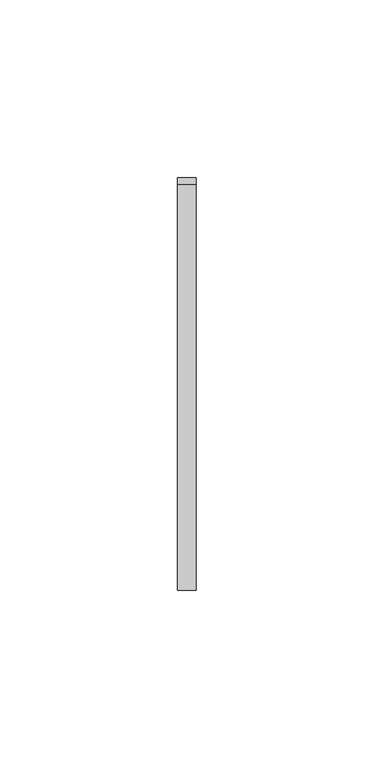
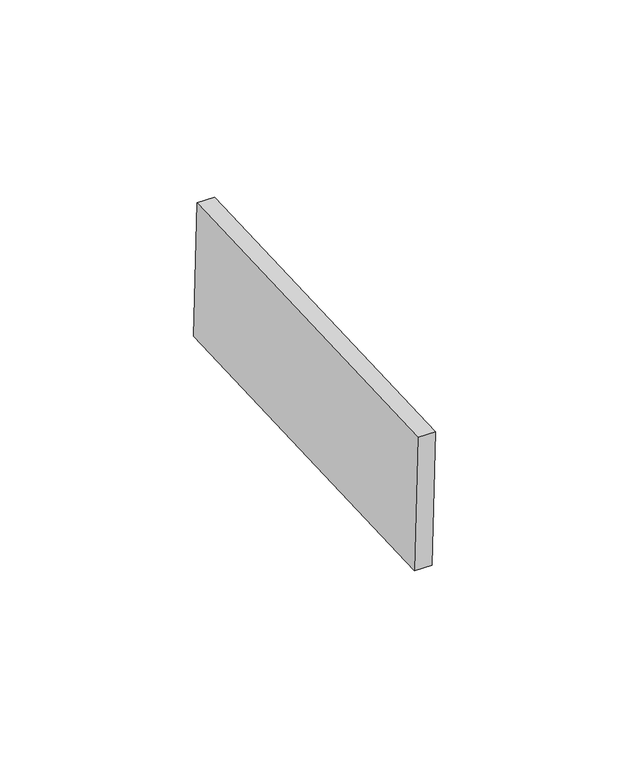
"""IFC4 building model written with IfcOpenShell, lengths in millimetres: proxy geometry, Inner panel:Inner panel:1:Inner panel:1 : Inner panel:Inner panel:300324:2:Inner panel:1:Inner panel:1 : Inner panel:Inner panel:300324:2 : Inner panel:Inner panel:1:Inner panel:1 : Inner panel:Inner panel:300324:300043:65 : Inner panel:Inner panel:1:Inner panel:1 : Inner panel:Inner panel:300324:2:Inner panel:1:Inner panel:1 : Inner panel:Inner panel:300324:2 : Inner panel:Inner panel:1:Inner panel:1 : Inner panel:Inner panel:300324:300043:308120."""

from ifc_helpers import new_model, si_unit, frame, origin, place, context, project, spatial, polyline, outline, extrude, source, transform, mapped, element, save


def generic_models_1821906e(model_context):
    return source(origin(), model_context, "Body", "SweptSolid", [
        extrude(outline(polyline([(0.0, -114.2999999), (0.0, 0.0), (5.2138089, 0.0), (5.2138089, -114.2999999), (0.0, -114.2999999)])), frame((593530.195117, -569718.1460118, 8742.3617848), z_axis=(0.0, -0.04163054471215927, 0.9991330730923529), x_axis=(-1.0, 0.0, 0.0)), (0.0, 0.0, 1.0), 43.2233908),
    ])


if __name__ == "__main__":
    model = new_model("IFC4")
    model_context = context("Model", 3, world=origin())
    ifc_project = project(units=[si_unit("LENGTHUNIT", "METRE", prefix="MILLI")], contexts=[model_context])
    site = spatial("IfcSite", under=ifc_project)
    building = spatial("IfcBuilding", under=site)
    placement = place(None, origin())
    generic_models_shape = generic_models_1821906e(model_context)
    element("IfcBuildingElementProxy", 1, Name="Inner panel:Inner panel:1:Inner panel:1 : Inner panel:Inner panel:300324:2:Inner panel:1:Inner panel:1 : Inner panel:Inner panel:300324:2 : Inner panel:Inner panel:1:Inner panel:1 : Inner panel:Inner panel:300324:300043:65 : Inner panel:Inner panel:1:Inner panel:1 : Inner panel:Inner panel:300324:2:Inner panel:1:Inner panel:1 : Inner panel:Inner panel:300324:2 : Inner panel:Inner panel:1:Inner panel:1 : Inner panel:Inner panel:300324:300043:308120", ObjectType="Inner panel:Inner panel:1:Inner panel:1 : Inner panel:Inner panel:300324:2:Inner panel:1:Inner panel:1 : Inner panel:Inner panel:300324:2 : Inner panel:Inner panel:1:Inner panel:1 : Inner panel:Inner panel:300324:300043:65 : Inner panel:Inner panel:1:Inner panel:1 : Inner panel:Inner panel:300324:2:Inner panel:1:Inner panel:1 : Inner panel:Inner panel:300324:2 : Inner panel:Inner panel:1:Inner panel:1 : Inner panel:Inner panel:300324:300043:308120", at=placement, inside=building, context=model_context, shape_type="MappedRepresentation", body=[
        mapped(generic_models_shape, transform((0.0, 0.0, 0.0), x_axis=(1.0, 0.0, 0.0), y_axis=(0.0, 1.0, 0.0), z_axis=(0.0, 0.0, 1.0))),
    ])
    save(model, "model.ifc")

# Revit data of these elements
# Type "Inner panel:Inner panel:1:Inner panel:1 : Inner panel:Inner panel:300324:2:Inner panel:1:Inner panel:1 : Inner panel:Inner panel:300324:2 : Inner panel:Inner panel:1:Inner panel:1 : Inner panel:Inner panel:300324:300043:65 : Inner panel:Inner panel:1:Inner panel:1 : Inner panel:Inner panel:300324:2:Inner panel:1:Inner panel:1 : Inner panel:Inner panel:300324:2 : Inner panel:Inner panel:1:Inner panel:1 : Inner panel:Inner panel:300324:300043:308120"
#   NameOverride = "Inner panel:Inner panel:1:Inner panel:1 : Inner panel:Inner panel:300324:2:Inner panel:1:Inner panel:1 : Inner panel:Inner panel:300324:2 : Inner panel:Inner panel:1:Inner panel:1 : Inner panel:Inner panel:300324:300043:308120"
#   ObjectTypeOverride = "Inner panel:1:Inner panel:1 : Inner panel:Inner panel:300324:2 : Inner panel:Inner panel:1:Inner panel:1 : Inner panel:Inner panel:300324:300043"
#   Reference = "Inner panel"
#   Tag = "308120"
# Element 1 (IfcBuildingElementProxy, "Inner panel:Inner panel:1:Inner panel:1 : Inner panel:Inner panel:300324:2:Inner panel:1:Inner panel:1 : Inner panel:Inner panel:300324:2 : Inner panel:Inner panel:1:Inner panel:1 : Inner panel:Inner panel:300324:300043:65 : Inner panel:Inner panel:1:Inner panel:1 : Inner panel:Inner panel:300324:2:Inner panel:1:Inner panel:1 : Inner panel:Inner panel:300324:2 : Inner panel:Inner panel:1:Inner panel:1 : Inner panel:Inner panel:300324:300043:308120")
#   Materials on its faces: "SLIDING CLIP"
# Materials
#   "SLIDING CLIP": class "Generic", colour RGB 120 120 120, transparency 0, Cost = 0
